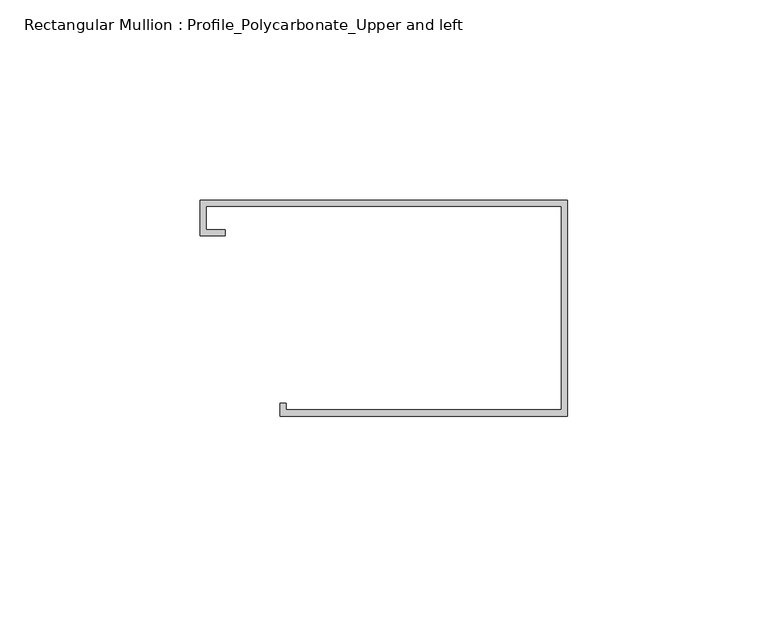
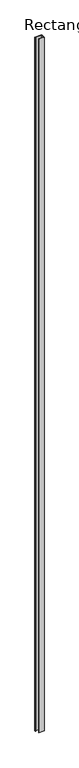
"""IFC4 building model written with IfcOpenShell, lengths in millimetres: member geometry, Rectangular Mullion : Profile_Polycarbonate_Upper and left."""

from ifc_helpers import new_model, si_unit, frame, origin, place, context, project, spatial, polyline, outline, extrude, source, transform, mapped, element, save


def rectangular_mullion_profile_polycarbonate_upper_and_left_172cc64e(model_context):
    return source(origin(), model_context, "Body", "SweptSolid", [
        extrude(outline(polyline([(0.0, 28.984575), (0.0, -25.015825), (-71.9836, -25.015825), (-71.9836, -21.840825), (-70.3961, -21.840825), (-70.3961, -23.428325), (-1.5875, -23.428325), (-1.5875, 27.397075), (-90.4113, 27.397075), (-90.4113, 21.580475), (-85.6488, 21.580475), (-85.6488, 19.992975), (-91.9988, 19.992975), (-91.9988, 28.984575), (0.0, 28.984575)])), frame((0.0, 0.0, -9863.2899), z_axis=(0.0, 0.0, 1.0), x_axis=(1.0, 0.0, 0.0)), (0.0, 0.0, 1.0), 9863.2899),
    ])


if __name__ == "__main__":
    model = new_model("IFC4")
    model_context = context("Model", 3, world=origin())
    ifc_project = project(units=[si_unit("LENGTHUNIT", "METRE", prefix="MILLI")], contexts=[model_context])
    site = spatial("IfcSite", under=ifc_project)
    building = spatial("IfcBuilding", under=site)
    placement = place(None, origin())
    rectangular_mullion_profile_polycarbonate_upper_and_left_shape = rectangular_mullion_profile_polycarbonate_upper_and_left_172cc64e(model_context)
    element("IfcMember", 1, ObjectType="Rectangular Mullion : Profile_Polycarbonate_Upper and left", at=placement, inside=building, context=model_context, shape_type="MappedRepresentation", body=[
        mapped(rectangular_mullion_profile_polycarbonate_upper_and_left_shape, transform((0.0, 0.0, 0.0), x_axis=(1.0, 0.0, 0.0), y_axis=(0.0, 1.0, 0.0), z_axis=(0.0, 0.0, 1.0))),
    ])
    save(model, "model.ifc")

# Revit data of these elements
# Type "Rectangular Mullion : Profile_Polycarbonate_Upper and left"
#   built-in parameter 1007322 = 0.177167 (stored number, unit not read)
#   built-in parameter 1007321 = 0.00520833 (stored number, unit not read)
#   built-in parameter 1007320 = 0 (stored number, unit not read)
